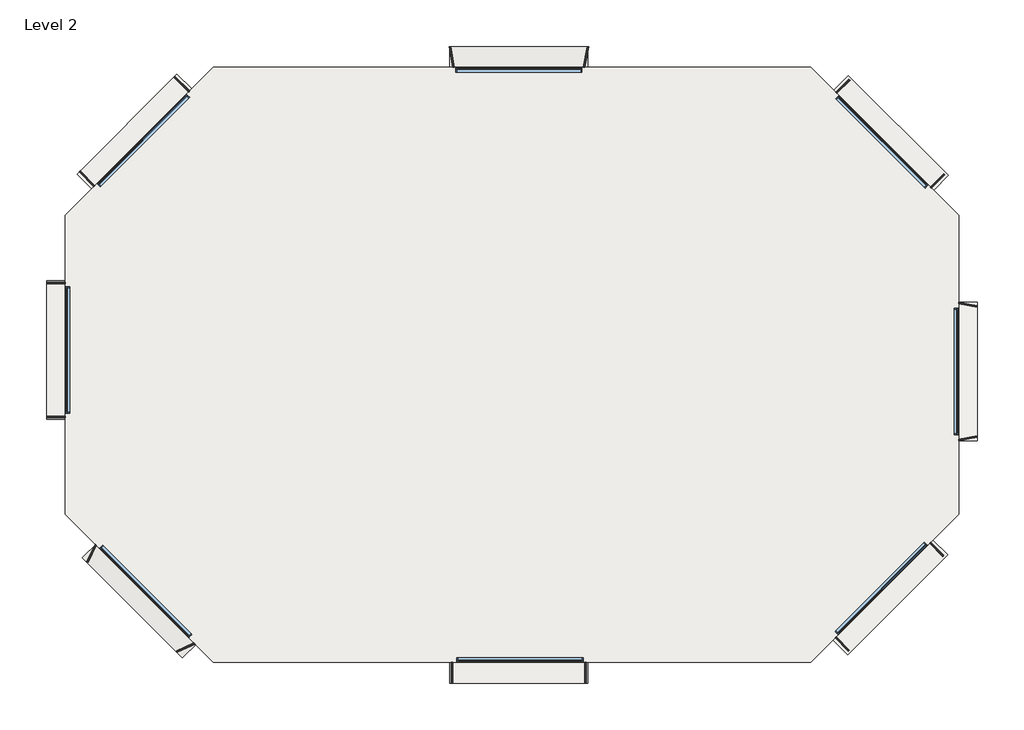
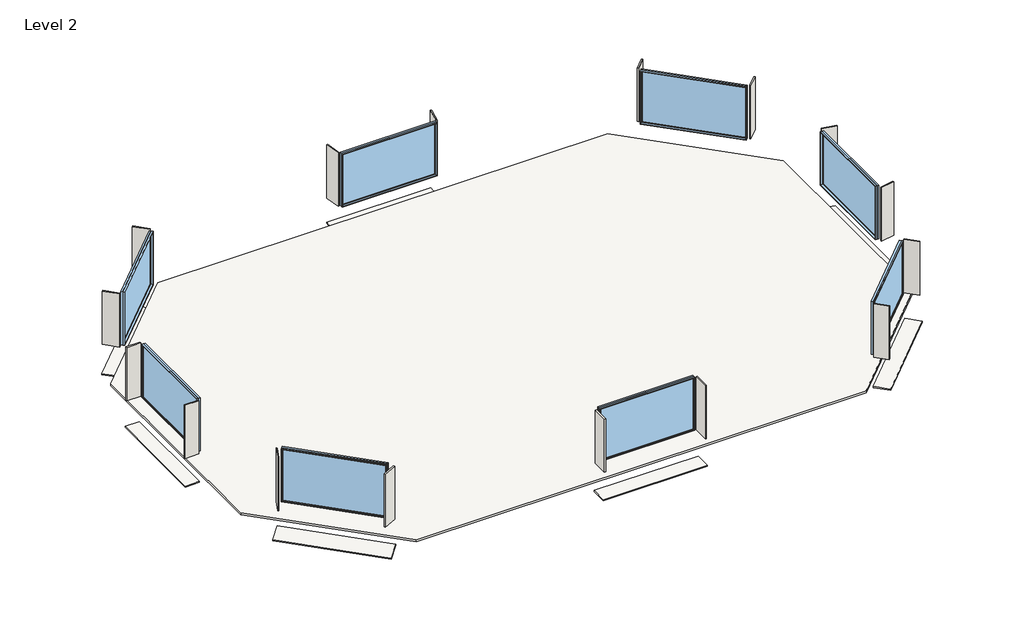
# One storey: 16 walls, 8 roofs, 8 windows, 1 slab.
"""IFC4 building model written with IfcOpenShell, lengths in millimetres."""

import ifcopenshell
import ifcopenshell.guid

model = None  # the IFC model being written
_history = None  # IfcOwnerHistory: only IFC2X3 demands one
_inside = {}  # id of a spatial element -> (the spatial element, [elements in it])
_under = {}  # id of a project, library or spatial element -> (it, [spatial elements below it])
_declared = {}  # id of a project -> (the project, [libraries it declares])
_typed = {}  # id of a type object -> (the type object, [elements of that type])
_made_of = {}  # id of a material, layer set ... -> (it, [elements and type objects made of it])


def new_model(schema):
    """Start an empty IFC model of exactly this schema.

    Asked for "IFC4X3", IfcOpenShell would pick the latest addendum, in which some entities
    have other attributes; the version numbers below select the first issue.
    IFC2X3 requires an IfcOwnerHistory on every rooted entity: one is made here for all.
    """
    global model, _history
    if schema == "IFC4X3":
        model = ifcopenshell.file(schema_version=(4, 3, 0, 0))
    else:
        model = ifcopenshell.file(schema=schema)
    _inside.clear()
    _under.clear()
    _declared.clear()
    _typed.clear()
    _made_of.clear()
    _history = None
    if model.schema == "IFC2X3":
        org = make("IfcOrganization", Name="unknown")
        user = make(
            "IfcPersonAndOrganization",
            ThePerson=make("IfcPerson", FamilyName="unknown"),
            TheOrganization=org,
        )
        app = make(
            "IfcApplication",
            ApplicationDeveloper=org,
            Version="unknown",
            ApplicationFullName="unknown",
            ApplicationIdentifier="unknown",
        )
        _history = make(
            "IfcOwnerHistory",
            OwningUser=user,
            OwningApplication=app,
            ChangeAction="ADDED",
            CreationDate=0,
        )
    return model


def make(cls, **values):
    """One entity of the class cls with the attributes given. An attribute that is None is left unset."""
    return model.create_entity(
        cls, **{name: value for name, value in values.items() if value is not None}
    )


def rooted(cls, **values):
    """An entity with a GlobalId (a new one), such as an element, a storey or a relation."""
    return make(cls, GlobalId=ifcopenshell.guid.new(), OwnerHistory=_history, **values)


def si_unit(unit_type, name, prefix=None):
    """IfcSIUnit, for example si_unit("LENGTHUNIT", "METRE", prefix="MILLI")."""
    return make("IfcSIUnit", UnitType=unit_type, Prefix=prefix, Name=name)


def assignment(units):
    """IfcUnitAssignment: the units of a project."""
    return None if units is None else make("IfcUnitAssignment", Units=units)


def point(xyz):
    """IfcCartesianPoint."""
    return None if xyz is None else make("IfcCartesianPoint", Coordinates=xyz)


def direction(xyz):
    """IfcDirection."""
    return None if xyz is None else make("IfcDirection", DirectionRatios=xyz)


def frame(location, z_axis=None, x_axis=None):
    """IfcAxis2Placement3D, a coordinate frame: its origin and axes. An axis left out is left unset."""
    return make(
        "IfcAxis2Placement3D",
        Location=point(location),
        Axis=direction(z_axis),
        RefDirection=direction(x_axis),
    )


def origin():
    """The frame at (0, 0, 0) with its axes left unset."""
    return frame((0.0, 0.0, 0.0))


def place(relative_to, where):
    """IfcLocalPlacement: puts the frame where relative to a parent placement (None: the world)."""
    return make(
        "IfcLocalPlacement", PlacementRelTo=relative_to, RelativePlacement=where
    )


def context(
    kind, dimensions, precision=None, world=None, true_north=None, identifier=None
):
    """IfcGeometricRepresentationContext, for example the 3D "Model" context."""
    return make(
        "IfcGeometricRepresentationContext",
        ContextIdentifier=identifier,
        ContextType=kind,
        CoordinateSpaceDimension=dimensions,
        Precision=precision,
        WorldCoordinateSystem=world,
        TrueNorth=true_north,
    )


def project(units=None, contexts=None):
    """IfcProject with its units and contexts."""
    return rooted(
        "IfcProject",
        Name="project",
        RepresentationContexts=contexts,
        UnitsInContext=assignment(units),
    )


def spatial(cls, under=None, at=None, **own):
    """A site, building, storey or space (cls), placed at a placement, below another one or the project."""
    s = rooted(cls, ObjectPlacement=at, **own)
    if under is not None:
        _under.setdefault(under.id(), (under, []))[1].append(s)
    return s


def polyline(points):
    """IfcPolyline through the points."""
    return make("IfcPolyline", Points=[point(p) for p in points])


def outline(outer, holes=None, kind="AREA"):
    """IfcArbitraryClosedProfileDef: a profile drawn as a closed curve; with holes, ...WithVoids."""
    if holes is None:
        return make("IfcArbitraryClosedProfileDef", ProfileType=kind, OuterCurve=outer)
    return make(
        "IfcArbitraryProfileDefWithVoids",
        ProfileType=kind,
        OuterCurve=outer,
        InnerCurves=holes,
    )


def extrude(swept, where, along, depth):
    """IfcExtrudedAreaSolid: the profile swept, set in the frame where, extruded along a direction by depth."""
    return make(
        "IfcExtrudedAreaSolid",
        SweptArea=swept,
        Position=where,
        ExtrudedDirection=direction(along),
        Depth=depth,
    )


def shape(context_of_items, identifier, shape_type, items):
    """IfcShapeRepresentation: the items that make up one representation, for example the "Body"."""
    return make(
        "IfcShapeRepresentation",
        ContextOfItems=context_of_items,
        RepresentationIdentifier=identifier,
        RepresentationType=shape_type,
        Items=items,
    )


def source(mapping_origin, context_of_items, identifier, shape_type, items):
    """IfcRepresentationMap: a shape defined once, which mapped items show again and again."""
    return make(
        "IfcRepresentationMap",
        MappingOrigin=mapping_origin,
        MappedRepresentation=shape(context_of_items, identifier, shape_type, items),
    )


def transform(
    local_origin,
    x_axis=None,
    y_axis=None,
    z_axis=None,
    scale=None,
    scale2=None,
    scale3=None,
    uniform=True,
):
    """IfcCartesianTransformationOperator3D, or its non-uniform kind. x_axis, y_axis, z_axis: its Axis1, 2, 3."""
    if uniform:
        return make(
            "IfcCartesianTransformationOperator3D",
            Axis1=direction(x_axis),
            Axis2=direction(y_axis),
            LocalOrigin=point(local_origin),
            Scale=scale,
            Axis3=direction(z_axis),
        )
    return make(
        "IfcCartesianTransformationOperator3DnonUniform",
        Axis1=direction(x_axis),
        Axis2=direction(y_axis),
        LocalOrigin=point(local_origin),
        Scale=scale,
        Axis3=direction(z_axis),
        Scale2=scale2,
        Scale3=scale3,
    )


def mapped(mapping_source, mapping_target):
    """IfcMappedItem: shows the shape of a source again, moved by a transform."""
    return make(
        "IfcMappedItem", MappingSource=mapping_source, MappingTarget=mapping_target
    )


def made_of(thing, what):
    """Note that an element or type object is made of a material, layer set ...; save() writes the relation."""
    if what is not None:
        _made_of.setdefault(what.id(), (what, []))[1].append(thing)
    return thing


def element(
    cls,
    number,
    at=None,
    inside=None,
    cuts=None,
    type_object=None,
    material=None,
    context=None,
    identifier="Body",
    shape_type=None,
    held_by="IfcProductDefinitionShape",
    body=None,
    shapes=None,
    **own,
):
    """One element of the class cls, such as IfcWall. Its Tag is "e" and its number.

    at: its placement. inside: the storey or other place that contains it. cuts: it is an
    opening in that element (IfcRelVoidsElement). A single representation is given by context,
    identifier, shape_type and body (its items); several are given by shapes. held_by: the class
    of the entity that holds the representations. save() writes the other relations.
    """
    e = rooted(cls, Tag="e%d" % number, ObjectPlacement=at, **own)
    if body is not None:
        shapes = [shape(context, identifier, shape_type, body)]
    if shapes is not None:
        e.Representation = make(held_by, Representations=shapes)
    if inside is not None:
        _inside.setdefault(inside.id(), (inside, []))[1].append(e)
    if cuts is not None:
        rooted(
            "IfcRelVoidsElement", RelatingBuildingElement=cuts, RelatedOpeningElement=e
        )
    if type_object is not None:
        _typed.setdefault(type_object.id(), (type_object, []))[1].append(e)
    return made_of(e, material)


def aggregate(whole, parts):
    """IfcRelAggregates: a whole, such as a stair, and the parts it consists of."""
    return rooted("IfcRelAggregates", RelatingObject=whole, RelatedObjects=parts)


def save(model, path):
    """Write the relations noted so far, then the file.

    IfcRelAggregates (storeys below a building ...), IfcRelContainedInSpatialStructure (elements
    in a storey), IfcRelDefinesByType, IfcRelAssociatesMaterial and IfcRelDeclares: one each for
    every whole, place, type object, material and project.
    """
    for whole, parts in _under.values():
        aggregate(whole, parts)
    for where, things in _inside.values():
        rooted(
            "IfcRelContainedInSpatialStructure",
            RelatedElements=things,
            RelatingStructure=where,
        )
    for kind, things in _typed.values():
        rooted("IfcRelDefinesByType", RelatedObjects=things, RelatingType=kind)
    for what, things in _made_of.values():
        rooted("IfcRelAssociatesMaterial", RelatedObjects=things, RelatingMaterial=what)
    for by, libraries in _declared.values():
        rooted("IfcRelDeclares", RelatingContext=by, RelatedDefinitions=libraries)
    model.write(path)


def m_fixed_2500x_4228mm_fd5e51e7(model_context):
    return source(origin(), model_context, "Body", "SweptSolid", [
        extrude(outline(polyline([(-2050.8, 54.2), (2050.8, 54.2), (2050.8, 42.2), (-2050.8, 42.2), (-2050.8, 54.2)])), frame((0.0, 0.0, 368.0), z_axis=(0.0, 0.0, 1.0), x_axis=(1.0, 0.0, 0.0)), (0.0, 0.0, 1.0), 2374.0),
        extrude(outline(polyline([(2786.0, -2094.8), (324.0, -2094.8), (324.0, 2094.8), (2786.0, 2094.8), (2786.0, -2094.8)]), holes=[polyline([(2742.0, -2050.8), (2742.0, 2050.8), (368.0, 2050.8), (368.0, -2050.8), (2742.0, -2050.8)])]), frame((0.0, 26.2, 0.0), z_axis=(0.0, 1.0, 0.0), x_axis=(0.0, 0.0, 1.0)), (0.0, 0.0, 1.0), 44.0),
        extrude(outline(polyline([(2805.0, -2113.8), (305.0, -2113.8), (305.0, 2113.8), (2805.0, 2113.8), (2805.0, -2113.8)]), holes=[polyline([(2786.0, -2094.8), (2786.0, 2094.8), (324.0, 2094.8), (324.0, -2094.8), (2786.0, -2094.8)])]), frame((0.0, 26.2, 0.0), z_axis=(0.0, 1.0, 0.0), x_axis=(0.0, 0.0, 1.0)), (0.0, 0.0, 1.0), 63.0),
        extrude(outline(polyline([(2805.0, -2113.8), (305.0, -2113.8), (305.0, 2113.8), (2805.0, 2113.8), (2805.0, -2113.8)]), holes=[polyline([(2773.0, -2081.8), (2773.0, 2081.8), (337.0, 2081.8), (337.0, -2081.8), (2773.0, -2081.8)])]), frame((0.0, -63.2, 0.0), z_axis=(0.0, 1.0, 0.0), x_axis=(0.0, 0.0, 1.0)), (0.0, 0.0, 1.0), 89.4),
    ])


model = new_model("IFC4")

# Units and contexts
model_context = context("Model", 3, world=origin())
ifc_project = project(units=[si_unit("LENGTHUNIT", "METRE", prefix="MILLI")], contexts=[model_context])

# Site, building, storey
site = spatial("IfcSite", under=ifc_project)
building = spatial("IfcBuilding", under=site)
storey = spatial("IfcBuildingStorey", under=building, Name="Level 2", Elevation=3962.4)

# Roofs
placement = place(None, origin())
element("IfcRoof", 1, ObjectType="Generic - 125mm shading", at=placement, inside=storey, context=model_context, shape_type="SweptSolid", body=[
    extrude(outline(polyline([(18552.7836697, -8602.5147149), (23180.3836697, -8602.5147149), (23180.3836697, -9302.5147149), (18552.7836697, -9302.5147149), (18552.7836697, -8602.5147149)])), frame((0.0, 0.0, 3450.0), z_axis=(0.0, 0.0, 1.0), x_axis=(1.0, 0.0, 0.0)), (0.0, 0.0, 1.0), 50.0),
])
element("IfcRoof", 2, ObjectType="Generic - 125mm shading", at=placement, inside=storey, context=model_context, shape_type="SweptSolid", body=[
    extrude(outline(polyline([(11296.9802217, 3500.7713306), (11996.9802217, 3624.2002171), (11996.9802217, 3573.4288865), (11296.9802217, 3450.0), (11296.9802217, 3500.7713306)])), frame((18552.7836697, 0.0, 0.0), z_axis=(1.0, 0.0, 0.0), x_axis=(0.0, 1.0, 0.0)), (0.0, 0.0, 1.0), 4627.6),
])
element("IfcRoof", 3, ObjectType="Generic - 125mm shading", at=placement, inside=storey, context=model_context, shape_type="SweptSolid", body=[
    extrude(outline(polyline([(34745.7885808, 7190.4058824), (31403.3995039, 10532.7949592), (31895.6627273, 11025.0581826), (35238.0518042, 7682.6691057), (34745.7885808, 7190.4058824)])), frame((0.0, 0.0, 3400.0), z_axis=(0.0, 0.0, 1.0), x_axis=(1.0, 0.0, 0.0)), (0.0, 0.0, 1.0), 50.0),
])
element("IfcRoof", 4, ObjectType="Generic - 125mm shading", at=placement, inside=storey, context=model_context, shape_type="SweptSolid", body=[
    extrude(outline(polyline([(31379.6986616, -7862.0302949), (34722.0877385, -4519.641218), (35214.3509618, -5011.9044414), (31871.961885, -8354.2935183), (31379.6986616, -7862.0302949)])), frame((0.0, 0.0, 3400.0), z_axis=(0.0, 0.0, 1.0), x_axis=(1.0, 0.0, 0.0)), (0.0, 0.0, 1.0), 50.0),
])
element("IfcRoof", 5, ObjectType="Generic - 125mm shading", at=placement, inside=storey, context=model_context, shape_type="SweptSolid", body=[
    extrude(outline(polyline([(9921.2320547, 10578.9980348), (6578.8429778, 7236.6089579), (6086.5797544, 7728.8721813), (9428.9688313, 11071.2612582), (9921.2320547, 10578.9980348)])), frame((0.0, 0.0, 3400.0), z_axis=(0.0, 0.0, 1.0), x_axis=(1.0, 0.0, 0.0)), (0.0, 0.0, 1.0), 50.0),
])
element("IfcRoof", 6, ObjectType="Generic - 125mm shading", at=placement, inside=storey, context=model_context, shape_type="SweptSolid", body=[
    extrude(outline(polyline([(696.1653267, 410.636191), (0.0, 597.1731281), (0.0, 648.9369371), (696.1653267, 462.4), (696.1653267, 410.636191)])), frame((9609.1938628, -8454.6807564, 3962.4), z_axis=(-0.7071067811865483, 0.7071067811865468, 0.0), x_axis=(0.7071067811865468, 0.7071067811865483, 0.0)), (0.0, 0.0, 1.0), 4726.8519632),
])
element("IfcRoof", 7, ObjectType="Generic - 125mm shading", at=placement, inside=storey, context=model_context, shape_type="SweptSolid", body=[
    extrude(outline(polyline([(3390.77856, 36212.7617098), (3500.7713306, 35588.9617098), (3450.0, 35588.9617098), (3340.0072294, 36212.7617098), (3390.77856, 36212.7617098)])), frame((0.0, -1191.3598794, 0.0), z_axis=(0.0, 1.0, 0.0), x_axis=(0.0, 0.0, 1.0)), (0.0, 0.0, 1.0), 4627.6),
])
element("IfcRoof", 8, ObjectType="Generic - 125mm shading", at=placement, inside=storey, context=model_context, shape_type="SweptSolid", body=[
    extrude(outline(polyline([(5689.4667732, 4156.608734), (5689.4667732, -470.991266), (5065.6667732, -470.991266), (5065.6667732, 4156.608734), (5689.4667732, 4156.608734)])), frame((0.0, 0.0, 3450.0), z_axis=(0.0, 0.0, 1.0), x_axis=(1.0, 0.0, 0.0)), (0.0, 0.0, 1.0), 50.0),
])

# Slab
element("IfcSlab", 9, ObjectType="Generic Floor - 100mm", at=placement, inside=storey, context=model_context, shape_type="SweptSolid", body=[
    extrude(outline(polyline([(10639.2142415, 11296.9802217), (30639.2142415, 11296.9802217), (35588.9617098, 6347.2327534), (35588.9617098, -3652.7672466), (30639.2142415, -8602.5147149), (10639.2142415, -8602.5147149), (5689.4667732, -3652.7672466), (5689.4667732, 6347.2327534), (10639.2142415, 11296.9802217)])), frame((0.0, 0.0, 3862.4), z_axis=(0.0, 0.0, 1.0), x_axis=(1.0, 0.0, 0.0)), (0.0, 0.0, 1.0), 100.0),
])

# Walls
element("IfcWall", 10, ObjectType="Generic - Shading", at=placement, inside=storey, context=model_context, shape_type="SweptSolid", body=[
    extrude(outline(polyline([(18602.7836697, -9302.5147149), (18602.7836697, -8602.5147149), (18652.7836697, -8602.5147149), (18652.7836697, -9302.5147149), (18602.7836697, -9302.5147149)])), frame((0.0, 0.0, 4762.4), z_axis=(0.0, 0.0, 1.0), x_axis=(1.0, 0.0, 0.0)), (0.0, 0.0, 1.0), 2500.0),
])
element("IfcWall", 11, ObjectType="Generic - Shading", at=placement, inside=storey, context=model_context, shape_type="SweptSolid", body=[
    extrude(outline(polyline([(23080.3836697, -9302.5147149), (23080.3836697, -8602.5147149), (23130.3836697, -8602.5147149), (23130.3836697, -9302.5147149), (23080.3836697, -9302.5147149)])), frame((0.0, 0.0, 4762.4), z_axis=(0.0, 0.0, 1.0), x_axis=(1.0, 0.0, 0.0)), (0.0, 0.0, 1.0), 2500.0),
])
element("IfcWall", 12, ObjectType="Generic - Shading", at=placement, inside=storey, context=model_context, shape_type="SweptSolid", body=[
    extrude(outline(polyline([(18585.0110058, 11995.425315), (18708.1657203, 11296.9802217), (18657.3943897, 11296.9802217), (18535.7706182, 11986.7429062), (18585.0110058, 11995.425315)])), frame((0.0, 0.0, 4762.4), z_axis=(0.0, 0.0, 1.0), x_axis=(1.0, 0.0, 0.0)), (0.0, 0.0, 1.0), 2500.0),
])
element("IfcWall", 13, ObjectType="Generic - Shading", at=placement, inside=storey, context=model_context, shape_type="SweptSolid", body=[
    extrude(outline(polyline([(23203.9773204, 11985.0795067), (23070.2243687, 11296.9802217), (23019.2885339, 11296.9802217), (23154.8959612, 11994.6199564), (23203.9773204, 11985.0795067)])), frame((0.0, 0.0, 4762.4), z_axis=(0.0, 0.0, 1.0), x_axis=(1.0, 0.0, 0.0)), (0.0, 0.0, 1.0), 2500.0),
])
element("IfcWall", 14, ObjectType="Generic - Shading", at=placement, inside=storey, context=model_context, shape_type="SweptSolid", body=[
    extrude(outline(polyline([(31949.4844771, 10868.8964063), (31508.391267, 10427.8031962), (31473.035928, 10463.1585352), (31914.1291381, 10904.2517453), (31949.4844771, 10868.8964063)])), frame((0.0, 0.0, 4762.4), z_axis=(0.0, 0.0, 1.0), x_axis=(1.0, 0.0, 0.0)), (0.0, 0.0, 1.0), 2500.0),
])
element("IfcWall", 15, ObjectType="Generic - Shading", at=placement, inside=storey, context=model_context, shape_type="SweptSolid", body=[
    extrude(outline(polyline([(35116.1711128, 7702.2097706), (34675.0779027, 7261.1165605), (34639.7225636, 7296.4718995), (35080.8157737, 7737.5651097), (35116.1711128, 7702.2097706)])), frame((0.0, 0.0, 4762.4), z_axis=(0.0, 0.0, 1.0), x_axis=(1.0, 0.0, 0.0)), (0.0, 0.0, 1.0), 2500.0),
])
element("IfcWall", 16, ObjectType="Generic - Shading", at=placement, inside=storey, context=model_context, shape_type="SweptSolid", body=[
    extrude(outline(polyline([(31890.4282957, -8233.487081), (31449.3350856, -7792.3938709), (31484.6904247, -7757.0385318), (31925.7836348, -8198.1317419), (31890.4282957, -8233.487081)])), frame((0.0, 0.0, 4762.4), z_axis=(0.0, 0.0, 1.0), x_axis=(1.0, 0.0, 0.0)), (0.0, 0.0, 1.0), 2500.0),
])
element("IfcWall", 17, ObjectType="Generic - Shading", at=placement, inside=storey, context=model_context, shape_type="SweptSolid", body=[
    extrude(outline(polyline([(35057.1149314, -5066.8004453), (34616.0217213, -4625.7072352), (34651.3770603, -4590.3518961), (35092.4702705, -5031.4451062), (35057.1149314, -5066.8004453)])), frame((0.0, 0.0, 4762.4), z_axis=(0.0, 0.0, 1.0), x_axis=(1.0, 0.0, 0.0)), (0.0, 0.0, 1.0), 2500.0),
])
element("IfcWall", 18, ObjectType="Generic - Shading", at=placement, inside=storey, context=model_context, shape_type="SweptSolid", body=[
    extrude(outline(polyline([(9356.6208838, 11004.3363576), (9851.5956306, 10509.3616108), (9816.2402916, 10474.0062717), (9321.2655447, 10968.9810185), (9356.6208838, 11004.3363576)])), frame((0.0, 0.0, 4762.4), z_axis=(0.0, 0.0, 1.0), x_axis=(1.0, 0.0, 0.0)), (0.0, 0.0, 1.0), 2500.0),
])
element("IfcWall", 19, ObjectType="Generic - Shading", at=placement, inside=storey, context=model_context, shape_type="SweptSolid", body=[
    extrude(outline(polyline([(6189.9342481, 7837.6497219), (6684.908995, 7342.6749751), (6649.5536559, 7307.319636), (6154.5789091, 7802.2943829), (6189.9342481, 7837.6497219)])), frame((0.0, 0.0, 4762.4), z_axis=(0.0, 0.0, 1.0), x_axis=(1.0, 0.0, 0.0)), (0.0, 0.0, 1.0), 2500.0),
])
element("IfcWall", 20, ObjectType="Generic - Shading", at=placement, inside=storey, context=model_context, shape_type="SweptSolid", body=[
    extrude(outline(polyline([(9422.3681472, -8225.9121729), (9995.4017447, -7958.7022181), (10033.0261106, -7996.326584), (9443.4990603, -8271.2275623), (9422.3681472, -8225.9121729)])), frame((0.0, 0.0, 4762.4), z_axis=(0.0, 0.0, 1.0), x_axis=(1.0, 0.0, 0.0)), (0.0, 0.0, 1.0), 2500.0),
])
element("IfcWall", 21, ObjectType="Generic - Shading", at=placement, inside=storey, context=model_context, shape_type="SweptSolid", body=[
    extrude(outline(polyline([(6412.8806073, -5240.6091093), (6687.7815855, -4651.0820589), (6725.4059515, -4688.7064249), (6458.1959966, -5261.7400224), (6412.8806073, -5240.6091093)])), frame((0.0, 0.0, 4762.4), z_axis=(0.0, 0.0, 1.0), x_axis=(1.0, 0.0, 0.0)), (0.0, 0.0, 1.0), 2500.0),
])
element("IfcWall", 22, ObjectType="Generic - Shading", at=placement, inside=storey, context=model_context, shape_type="SweptSolid", body=[
    extrude(outline(polyline([(36211.7856278, -1080.2032111), (35588.9617098, -1190.0238721), (35588.9617098, -1139.2525415), (36203.1032189, -1030.9628234), (36211.7856278, -1080.2032111)])), frame((0.0, 0.0, 4762.4), z_axis=(0.0, 0.0, 1.0), x_axis=(1.0, 0.0, 0.0)), (0.0, 0.0, 1.0), 2500.0),
])
element("IfcWall", 23, ObjectType="Generic - Shading", at=placement, inside=storey, context=model_context, shape_type="SweptSolid", body=[
    extrude(outline(polyline([(36203.1032189, 3275.8430645), (35588.9617098, 3384.1327826), (35588.9617098, 3434.9041132), (36211.7856278, 3325.0834522), (36203.1032189, 3275.8430645)])), frame((0.0, 0.0, 4762.4), z_axis=(0.0, 0.0, 1.0), x_axis=(1.0, 0.0, 0.0)), (0.0, 0.0, 1.0), 2500.0),
])
element("IfcWall", 24, ObjectType="Generic - Shading", at=placement, inside=storey, context=model_context, shape_type="SweptSolid", body=[
    extrude(outline(polyline([(5065.6667732, -370.991266), (5689.4667732, -370.991266), (5689.4667732, -420.991266), (5065.6667732, -420.991266), (5065.6667732, -370.991266)])), frame((0.0, 0.0, 4762.4), z_axis=(0.0, 0.0, 1.0), x_axis=(1.0, 0.0, 0.0)), (0.0, 0.0, 1.0), 2500.0),
])
element("IfcWall", 25, ObjectType="Generic - Shading", at=placement, inside=storey, context=model_context, shape_type="SweptSolid", body=[
    extrude(outline(polyline([(5065.6667732, 4106.608734), (5689.4667732, 4106.608734), (5689.4667732, 4056.608734), (5065.6667732, 4056.608734), (5065.6667732, 4106.608734)])), frame((0.0, 0.0, 4762.4), z_axis=(0.0, 0.0, 1.0), x_axis=(1.0, 0.0, 0.0)), (0.0, 0.0, 1.0), 2500.0),
])

# Windows
m_fixed_2500x_4228mm_shape = m_fixed_2500x_4228mm_fd5e51e7(model_context)
element("IfcWindow", 26, ObjectType="M_Fixed : 2500X 4228mm", at=placement, inside=storey, context=model_context, shape_type="MappedRepresentation", body=[
    mapped(m_fixed_2500x_4228mm_shape, transform((20907.1791073, -8513.3147149, 4457.4), x_axis=(-1.0, 0.0, 0.0), y_axis=(0.0, -1.0, 0.0), z_axis=(0.0, 0.0, 1.0))),
])
element("IfcWindow", 27, ObjectType="M_Fixed : 2500X 4228mm", at=placement, inside=storey, context=model_context, shape_type="MappedRepresentation", body=[
    mapped(m_fixed_2500x_4228mm_shape, transform((32987.5548042, -6128.0263025, 4457.4), x_axis=(-0.707106781186548, -0.7071067811865471, 0.0), y_axis=(0.7071067811865471, -0.707106781186548, 0.0), z_axis=(0.0, 0.0, 1.0))),
])
element("IfcWindow", 28, ObjectType="M_Fixed : 2500X 4228mm", at=placement, inside=storey, context=model_context, shape_type="MappedRepresentation", body=[
    mapped(m_fixed_2500x_4228mm_shape, transform((35499.7617098, 1122.4401206, 4457.4), x_axis=(0.0, -1.0, 0.0), y_axis=(1.0, 0.0, 0.0), z_axis=(0.0, 0.0, 1.0))),
])
element("IfcWindow", 29, ObjectType="M_Fixed : 2500X 4228mm", at=placement, inside=storey, context=model_context, shape_type="MappedRepresentation", body=[
    mapped(m_fixed_2500x_4228mm_shape, transform((33011.2556466, 8798.7909669, 4457.4), x_axis=(0.7071067811865468, -0.7071067811865483, 0.0), y_axis=(0.7071067811865483, 0.7071067811865468, 0.0), z_axis=(0.0, 0.0, 1.0))),
])
element("IfcWindow", 30, ObjectType="M_Fixed : 2500X 4228mm", at=placement, inside=storey, context=model_context, shape_type="MappedRepresentation", body=[
    mapped(m_fixed_2500x_4228mm_shape, transform((20866.5836697, 11207.7802217, 4457.4), x_axis=(1.0, 0.0, 0.0), y_axis=(0.0, 1.0, 0.0), z_axis=(0.0, 0.0, 1.0))),
])
element("IfcWindow", 31, ObjectType="M_Fixed : 2500X 4228mm", at=placement, inside=storey, context=model_context, shape_type="MappedRepresentation", body=[
    mapped(m_fixed_2500x_4228mm_shape, transform((8313.375912, 8844.9940424, 4457.4), x_axis=(0.7071067811865479, 0.707106781186547, 0.0), y_axis=(-0.707106781186547, 0.7071067811865479, 0.0), z_axis=(0.0, 0.0, 1.0))),
])
element("IfcWindow", 32, ObjectType="M_Fixed : 2500X 4228mm", at=placement, inside=storey, context=model_context, shape_type="MappedRepresentation", body=[
    mapped(m_fixed_2500x_4228mm_shape, transform((5778.6667732, 1842.808734, 4457.4), x_axis=(0.0, 1.0, 0.0), y_axis=(-1.0, 0.0, 0.0), z_axis=(0.0, 0.0, 1.0))),
])
element("IfcWindow", 33, ObjectType="M_Fixed : 2500X 4228mm", at=placement, inside=storey, context=model_context, shape_type="MappedRepresentation", body=[
    mapped(m_fixed_2500x_4228mm_shape, transform((8388.5493935, -6225.7020172, 4457.4), x_axis=(-0.707106781186546, 0.707106781186549, 0.0), y_axis=(-0.707106781186549, -0.707106781186546, 0.0), z_axis=(0.0, 0.0, 1.0))),
])

save(model, "model.ifc")

# Revit data of these elements
# Type "Generic - 125mm shading"
#   Layers, outside or top first: 50 mm no material (function 1)
# Type "Generic Floor - 100mm"
#   Function = 0
#   Layers, outside or top first: 100 mm no material (function 1)
# Type "Generic - Shading"
#   Layers, outside or top first: 50 mm no material (function 1)
# Type "M_Fixed : 2500X 4228mm"
#   Type Mark = "25"
#   Height = 2500 mm
#   Default Sill Height = 305 mm
#   Width = 4227.6 mm
#   Window Inset = 19 mm
#   Frame Exterior Material = Sash
#   Frame Interior Material = Sash
#   Glass Pane Material = Glass
#   Sash = Sash
#   Wall Closure = (empty or 0)
# Elements 1, 8 (IfcRoof, "Generic - 125mm shading")
#   built-in parameter 1001705 = 11.4829 (stored number, unit not read)
#   built-in parameter 1001701 = -1.6811 (stored number, unit not read)
#   built-in parameter 1001710 = 33615
#   Phase Created = New Construction
#   Materials on its faces: "Default Roof"
# Element 2 (IfcRoof, "Generic - 125mm shading")
#   built-in parameter 1001705 = 11.8904 (stored number, unit not read)
#   built-in parameter 1001701 = -1.6811 (stored number, unit not read)
#   built-in parameter 1001710 = 33615
#   Phase Created = New Construction
#   Materials on its faces: "Default Roof"
# Elements 3, 4, 5 (IfcRoof, "Generic - 125mm shading")
#   built-in parameter 1001705 = 11.3189 (stored number, unit not read)
#   built-in parameter 1001701 = -1.84514 (stored number, unit not read)
#   built-in parameter 1001710 = 33615
#   Phase Created = New Construction
#   Materials on its faces: "Default Roof"
# Element 6 (IfcRoof, "Generic - 125mm shading")
#   built-in parameter 1001705 = 11.6528 (stored number, unit not read)
#   built-in parameter 1001701 = -1.51706 (stored number, unit not read)
#   built-in parameter 1001710 = 33615
#   Phase Created = New Construction
#   Materials on its faces: "Default Roof"
# Element 7 (IfcRoof, "Generic - 125mm shading")
#   built-in parameter 1001705 = 11.4855 (stored number, unit not read)
#   built-in parameter 1001701 = -1.6811 (stored number, unit not read)
#   built-in parameter 1001710 = 33615
#   Phase Created = New Construction
#   Materials on its faces: "Default Roof"
# Element 9 (IfcSlab, "Generic Floor - 100mm")
#   built-in parameter 1001955 = 0.785398 (stored number, unit not read)
#   Height Offset From Level = 0 mm
#   Phase Created = New Construction
#   Materials on its faces: "Default Floor"
# Elements 10, 11, 12, 13, 14, 15, 16, 17, 18, 19, 20, 21, 22, 23, 24, 25 (IfcWall, "Generic - Shading")
#   built-in parameter 1001111 = 800 mm
#   Top Offset = -662.4 mm
#   Base Offset = 800 mm
#   wall height = 2500 mm
#   Phase Created = New Construction
#   Base Constraint = Level 2
#   Top Constraint = Roof Level
#   Materials on its faces: "Default Wall"
# Element 26 (IfcWindow, "M_Fixed : 2500X 4228mm")
#   Mark = "23"
#   Phase Created = New Construction
#   Materials on its faces: "Sash", "Glass"
# Element 27 (IfcWindow, "M_Fixed : 2500X 4228mm")
#   Mark = "24"
#   Phase Created = New Construction
#   Materials on its faces: "Sash", "Glass"
# Element 28 (IfcWindow, "M_Fixed : 2500X 4228mm")
#   Mark = "26"
#   Phase Created = New Construction
#   Materials on its faces: "Sash", "Glass"
# Element 29 (IfcWindow, "M_Fixed : 2500X 4228mm")
#   Mark = "33"
#   Phase Created = New Construction
#   Materials on its faces: "Sash", "Glass"
# Element 30 (IfcWindow, "M_Fixed : 2500X 4228mm")
#   Mark = "34"
#   Phase Created = New Construction
#   Materials on its faces: "Sash", "Glass"
# Element 31 (IfcWindow, "M_Fixed : 2500X 4228mm")
#   Mark = "35"
#   Phase Created = New Construction
#   Materials on its faces: "Sash", "Glass"
# Element 32 (IfcWindow, "M_Fixed : 2500X 4228mm")
#   Mark = "36"
#   Phase Created = New Construction
#   Materials on its faces: "Sash", "Glass"
# Element 33 (IfcWindow, "M_Fixed : 2500X 4228mm")
#   Mark = "37"
#   Phase Created = New Construction
#   Materials on its faces: "Sash", "Glass"
# Materials
#   "Sash": class "Wood", colour RGB 136 99 55, transparency 0
#   "Glass": class "Glass", colour RGB 0 128 192, transparency 0.9, Description = "Soda Lime Glass", Cost = 0
#   "Default Roof": class "Miscellaneous", colour RGB 0 127 0, transparency 0, Cost = 0
#   "Default Floor": class "Miscellaneous", colour RGB 127 127 127, transparency 0, Cost = 0
#   "Default Wall": class "Miscellaneous", colour RGB 128 128 128, transparency 0, Cost = 0
# Room at (21789.452, 2355.414) mm, phase "New Construction", upper level "Level 2", upper offset 3962.4 mm, lower offset 0 mm
#   Number = "12"
#   Name = "Room"
